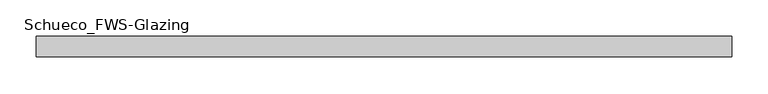
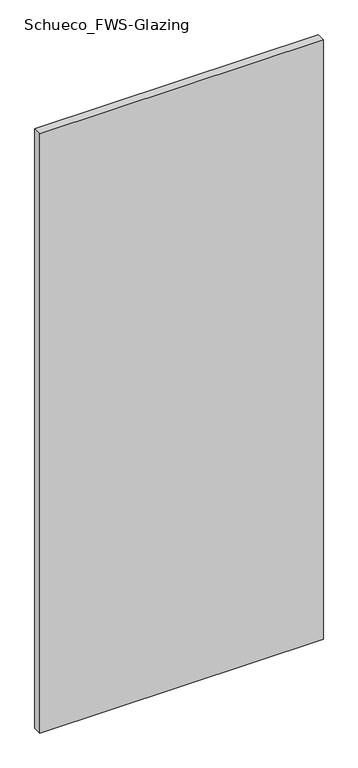
"""IFC4 building model written with IfcOpenShell, lengths in millimetres: plate geometry, Schueco_FWS-Glazing : HI_28mm_DoubGlz."""

from ifc_helpers import new_model, si_unit, origin, origin_with_axes, place, context, project, spatial, polyline, outline, extrude, source, transform, mapped, element, save


def schueco_fws_glazing_de60169a(model_context):
    return source(origin(), model_context, "Body", "SweptSolid", [
        extrude(outline(polyline([(476.5, -28.0), (-476.5, -28.0), (-476.5, 0.0), (476.5, 0.0), (476.5, -28.0)])), origin_with_axes(), (0.0, 0.0, 1.0), 2128.0),
    ])


if __name__ == "__main__":
    model = new_model("IFC4")
    model_context = context("Model", 3, world=origin())
    ifc_project = project(units=[si_unit("LENGTHUNIT", "METRE", prefix="MILLI")], contexts=[model_context])
    site = spatial("IfcSite", under=ifc_project)
    building = spatial("IfcBuilding", under=site)
    placement = place(None, origin())
    schueco_fws_glazing_shape = schueco_fws_glazing_de60169a(model_context)
    element("IfcPlate", 1, ObjectType="Schueco_FWS-Glazing : HI_28mm_DoubGlz", at=placement, inside=building, context=model_context, shape_type="MappedRepresentation", body=[
        mapped(schueco_fws_glazing_shape, transform((0.0, 0.0, 0.0), x_axis=(1.0, 0.0, 0.0), y_axis=(0.0, 1.0, 0.0), z_axis=(0.0, 0.0, 1.0))),
    ])
    save(model, "model.ifc")

# Revit data of these elements
# Type "Schueco_FWS-Glazing : HI_28mm_DoubGlz"
#   Model = "Double glazing 28mm"
#   Manufacturer = "Schueco International KG"
#   Analytic Construction = "<Keine Auswahl>"
#   Glazing thickness = 28 mm
#   FWS SI insert unit = no
#   FWS HI insert unit = yes
#   Glass = Glass
# Element 1 (IfcPlate, "Schueco_FWS-Glazing : HI_28mm_DoubGlz")
#   Materials on its faces: "Glass"
# Materials
#   "Glass": class "Glass", colour RGB 128 128 255, transparency 0.75, Description = "Soda Lime Glass", Cost = 0
